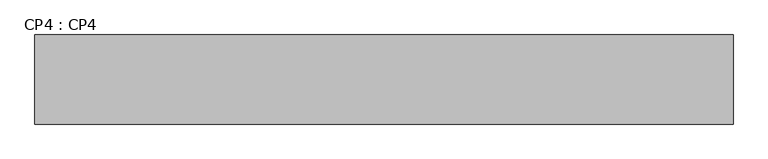
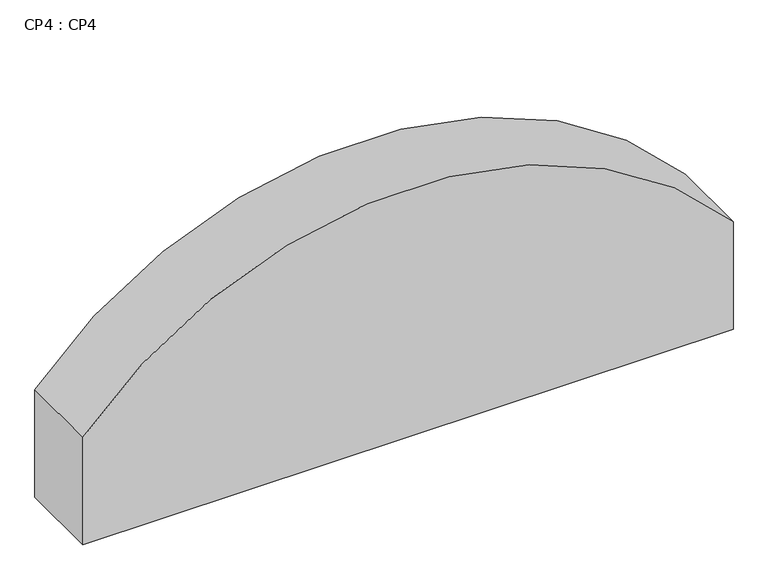
"""IFC4 building model written with IfcOpenShell, lengths in millimetres: beam geometry, CP4 : CP4."""

from ifc_helpers import new_model, si_unit, point, frame, frame_2d, origin, place, context, project, spatial, polyline, circle_curve, trimmed, segment, composite_curve, outline, extrude, source, transform, mapped, element, save


def cp4_cp4_5a1beb14(model_context):
    return source(origin(), model_context, "Body", "SweptSolid", [
        extrude(outline(composite_curve([segment(trimmed(circle_curve(frame_2d((12603.2870371, 32833.2245514)), 3096.7129629), [point((14620.0, 35183.2245514))], [point((14620.0, 30483.2245515))], False, "CARTESIAN"), True, "CONTINUOUS"), segment(polyline([(14620.0, 30483.2245515), (13800.0, 30483.2245515), (13800.0, 35183.2245514), (14620.0, 35183.2245514)]), True, "CONTINUOUS")], self_intersect=False)), frame((0.0, -100.2551788, 0.0), z_axis=(0.0, 1.0, 0.0), x_axis=(0.0, 0.0, 1.0)), (0.0, 0.0, 1.0), 599.9551778),
    ])


if __name__ == "__main__":
    model = new_model("IFC4")
    model_context = context("Model", 3, world=origin())
    ifc_project = project(units=[si_unit("LENGTHUNIT", "METRE", prefix="MILLI")], contexts=[model_context])
    site = spatial("IfcSite", under=ifc_project)
    building = spatial("IfcBuilding", under=site)
    placement = place(None, origin())
    cp4_cp4_shape = cp4_cp4_5a1beb14(model_context)
    element("IfcBeam", 1, ObjectType="CP4 : CP4", at=placement, inside=building, context=model_context, shape_type="MappedRepresentation", body=[
        mapped(cp4_cp4_shape, transform((0.0, 0.0, 0.0), x_axis=(1.0, 0.0, 0.0), y_axis=(0.0, 1.0, 0.0), z_axis=(0.0, 0.0, 1.0))),
    ])
    save(model, "model.ifc")
